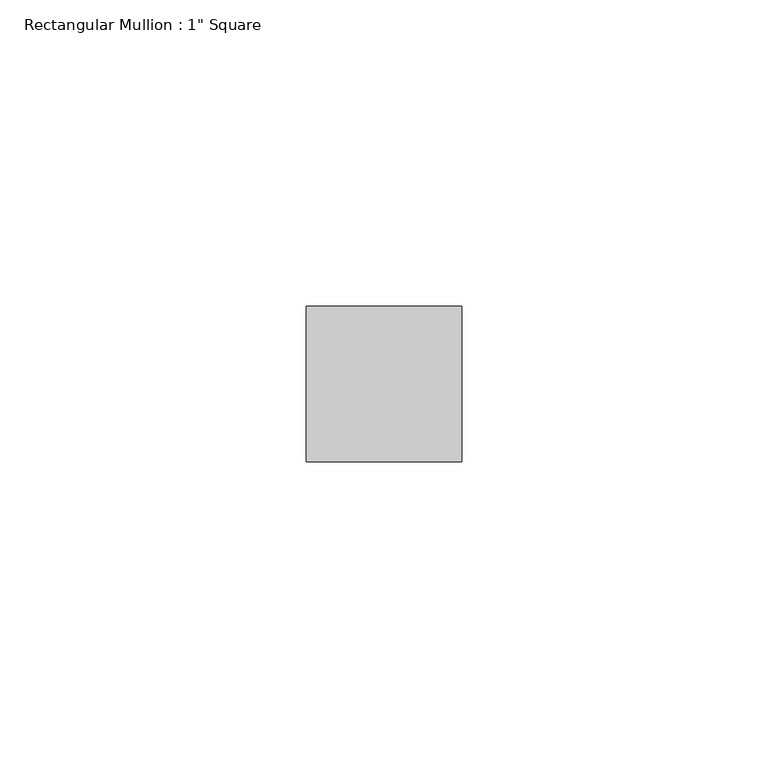
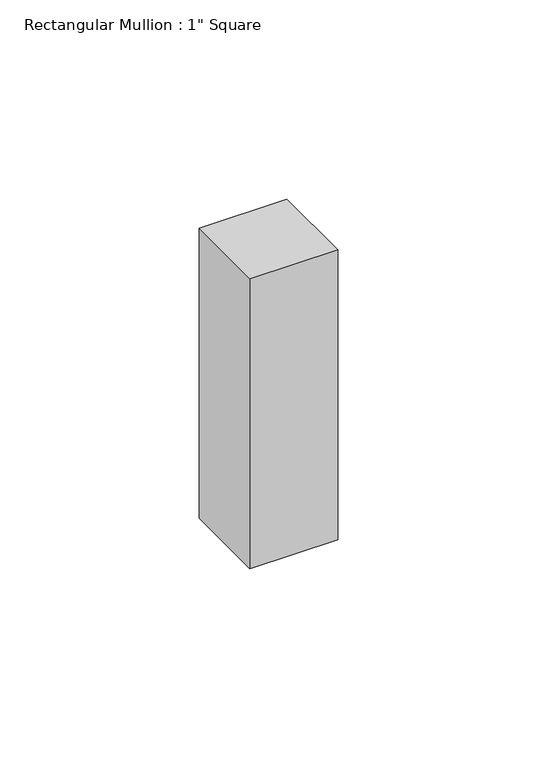
"""IFC4 building model written with IfcOpenShell, lengths in millimetres: member geometry."""

from ifc_helpers import new_model, si_unit, frame, origin, place, context, project, spatial, polyline, outline, extrude, source, transform, mapped, element, save


def member_a528e602(model_context):
    return source(origin(), model_context, "Body", "SweptSolid", [
        extrude(outline(polyline([(12.7, 12.7), (12.7, -12.7), (-12.7, -12.7), (-12.7, 12.7), (12.7, 12.7)])), frame((0.0, 0.0, -88.9), z_axis=(0.0, 0.0, 1.0), x_axis=(1.0, 0.0, 0.0)), (0.0, 0.0, 1.0), 88.9),
    ])


if __name__ == "__main__":
    model = new_model("IFC4")
    model_context = context("Model", 3, world=origin())
    ifc_project = project(units=[si_unit("LENGTHUNIT", "METRE", prefix="MILLI")], contexts=[model_context])
    site = spatial("IfcSite", under=ifc_project)
    building = spatial("IfcBuilding", under=site)
    placement = place(None, origin())
    member_shape = member_a528e602(model_context)
    element("IfcMember", 1, ObjectType="Rectangular Mullion : 1\" Square", at=placement, inside=building, context=model_context, shape_type="MappedRepresentation", body=[
        mapped(member_shape, transform((0.0, 0.0, 0.0), x_axis=(1.0, 0.0, 0.0), y_axis=(0.0, 1.0, 0.0), z_axis=(0.0, 0.0, 1.0))),
    ])
    save(model, "model.ifc")

# Revit data of these elements
# Type "Rectangular Mullion : 1\" Square"
#   built-in parameter 1007304 = 0.0833333 (stored number, unit not read)
#   built-in parameter 1007301 = 0.0416667 (stored number, unit not read)
#   built-in parameter 1007300 = 0.0416667 (stored number, unit not read)
# Element 1 (IfcMember, "Rectangular Mullion : 1\" Square")
#   Materials on its faces: "Metal - Aluminum"
# Materials
#   "Metal - Aluminum": class "Metal", colour RGB 247 247 247, transparency 0
